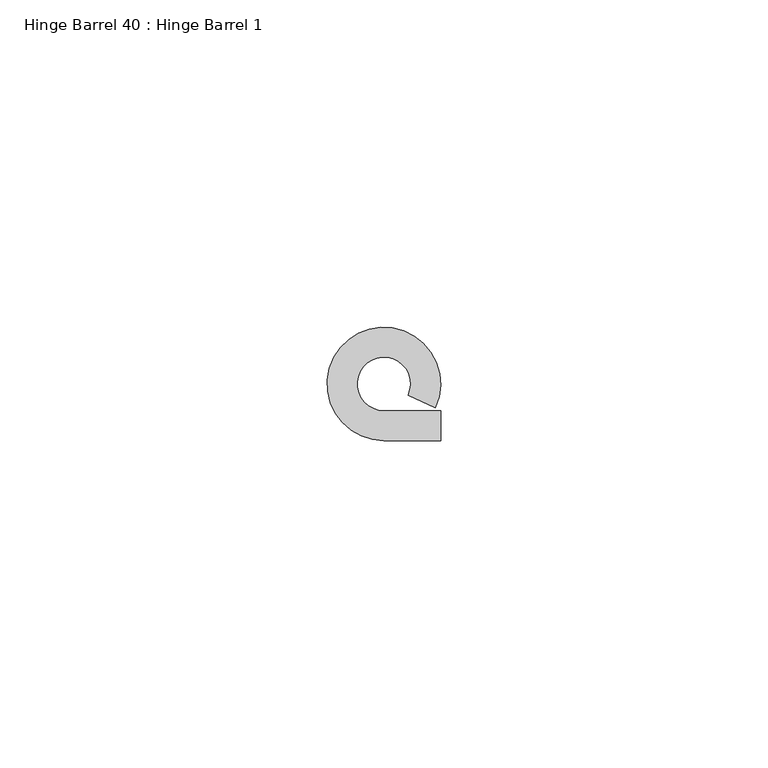
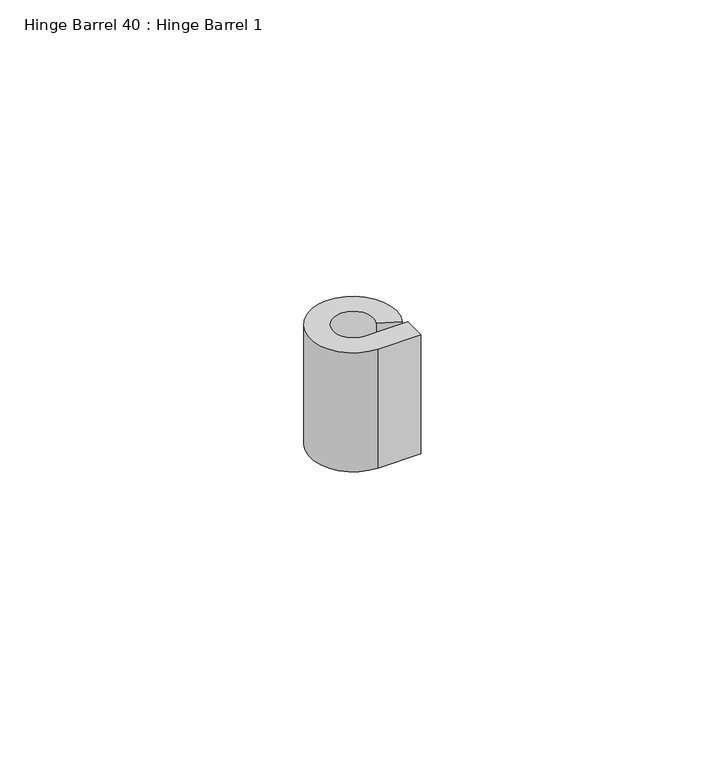
"""IFC4 building model written with IfcOpenShell, lengths in millimetres: proxy geometry, Hinge Barrel 40 : Hinge Barrel 1."""

from ifc_helpers import new_model, si_unit, point, frame, frame_2d, origin, place, context, project, spatial, polyline, circle_curve, trimmed, segment, composite_curve, outline, extrude, source, transform, mapped, element, save


def hinge_barrel_40_hinge_barrel_1_a2f6928c(model_context):
    return source(origin(), model_context, "Body", "SweptSolid", [
        extrude(outline(composite_curve([segment(polyline([(587323.2214739, -534104.7943841), (587327.7934739, -534104.7943841), (587327.7934739, -534109.3584466), (587319.1320739, -534109.3584466)]), True, "CONTINUOUS"), segment(trimmed(circle_curve(frame_2d((587319.1320739, -534100.7049841)), 8.6534625), [point((587319.1320739, -534109.3584466))], [point((587326.986084, -534104.3377433))], False, "CARTESIAN"), True, "CONTINUOUS"), segment(polyline([(587326.986084, -534104.3377433), (587322.8436736, -534102.421731)]), True, "CONTINUOUS"), segment(trimmed(circle_curve(frame_2d((587319.1320739, -534100.7049841)), 4.0894), [point((587322.8436736, -534102.421731))], [point((587319.1320739, -534104.7943841))], True, "CARTESIAN"), True, "CONTINUOUS"), segment(polyline([(587319.1320739, -534104.7943841), (587323.2214739, -534104.7943841)]), True, "CONTINUOUS")], self_intersect=False)), frame((0.0, 0.0, 412.75), z_axis=(0.0, 0.0, 1.0), x_axis=(1.0, 0.0, 0.0)), (0.0, 0.0, 1.0), 25.4),
    ])


if __name__ == "__main__":
    model = new_model("IFC4")
    model_context = context("Model", 3, world=origin())
    ifc_project = project(units=[si_unit("LENGTHUNIT", "METRE", prefix="MILLI")], contexts=[model_context])
    site = spatial("IfcSite", under=ifc_project)
    building = spatial("IfcBuilding", under=site)
    placement = place(None, origin())
    hinge_barrel_40_hinge_barrel_1_shape = hinge_barrel_40_hinge_barrel_1_a2f6928c(model_context)
    element("IfcBuildingElementProxy", 1, Name="Hinge Barrel 40 : Hinge Barrel 1", ObjectType="Hinge Barrel 40 : Hinge Barrel 1", at=placement, inside=building, context=model_context, shape_type="MappedRepresentation", body=[
        mapped(hinge_barrel_40_hinge_barrel_1_shape, transform((0.0, 0.0, 0.0), x_axis=(1.0, 0.0, 0.0), y_axis=(0.0, 1.0, 0.0), z_axis=(0.0, 0.0, 1.0))),
    ])
    save(model, "model.ifc")

# Revit data of these elements
# Element 1 (IfcBuildingElementProxy, "Hinge Barrel 40 : Hinge Barrel 1")
#   Materials on its faces: "6\"X6\" WELD-ON STL BUTT HINGE"
# Materials
#   "6\"X6\" WELD-ON STL BUTT HINGE": class "Metal", colour RGB 189 187 185, transparency 0, Description = "Carbon steel", Cost = 0
